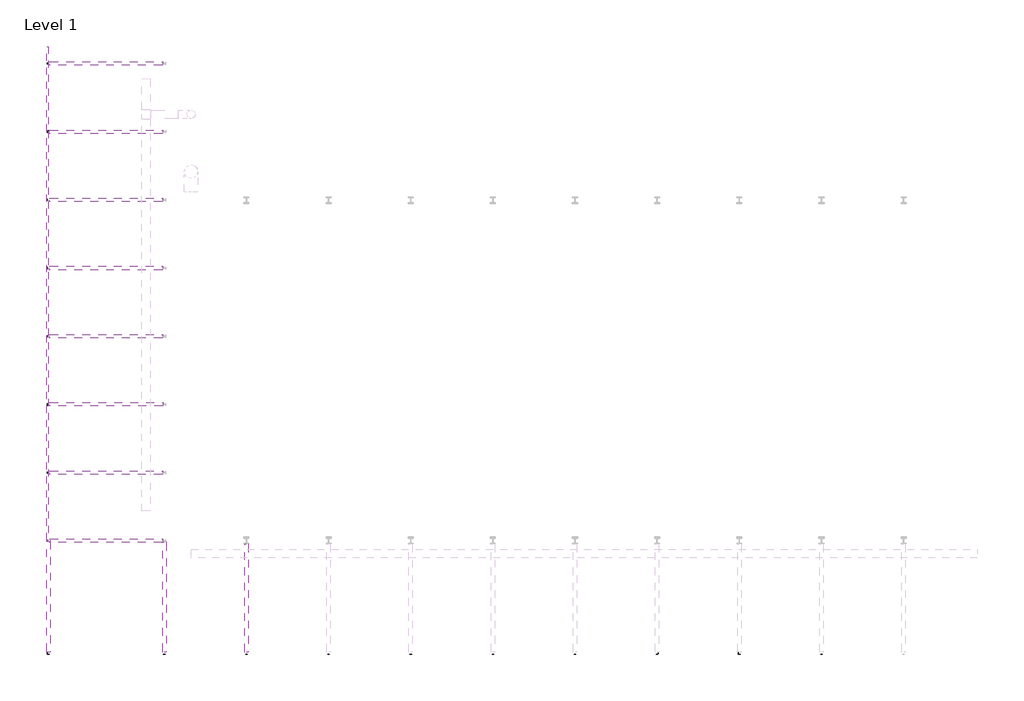
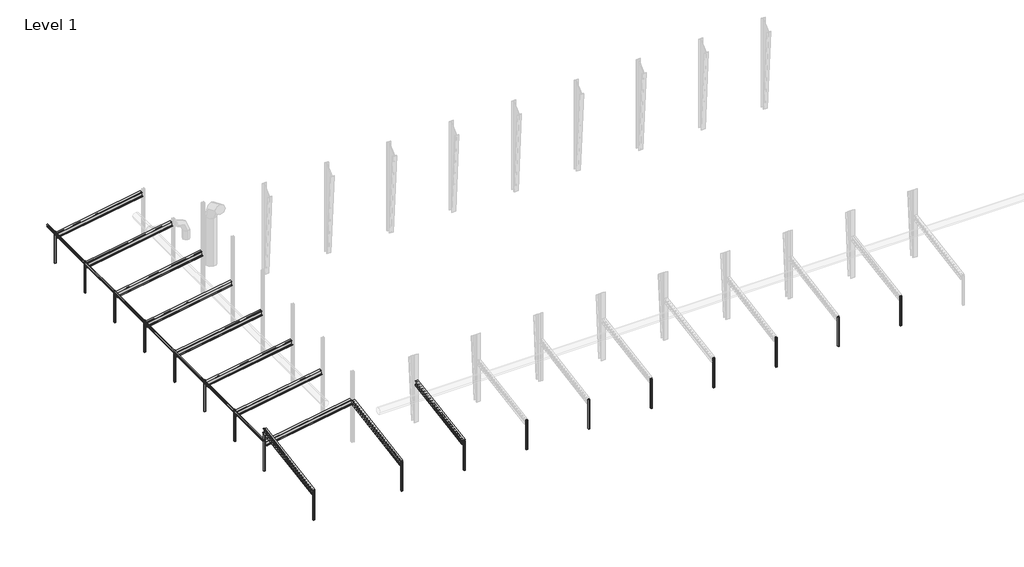
# One storey, part 1 of 3: 18 columns, 12 beams.
"""IFC4 building model written with IfcOpenShell, lengths in millimetres."""

import ifcopenshell
import ifcopenshell.guid

model = None  # the IFC model being written
_history = None  # IfcOwnerHistory: only IFC2X3 demands one
_inside = {}  # id of a spatial element -> (the spatial element, [elements in it])
_under = {}  # id of a project, library or spatial element -> (it, [spatial elements below it])
_declared = {}  # id of a project -> (the project, [libraries it declares])
_typed = {}  # id of a type object -> (the type object, [elements of that type])
_made_of = {}  # id of a material, layer set ... -> (it, [elements and type objects made of it])


def new_model(schema):
    """Start an empty IFC model of exactly this schema.

    Asked for "IFC4X3", IfcOpenShell would pick the latest addendum, in which some entities
    have other attributes; the version numbers below select the first issue.
    IFC2X3 requires an IfcOwnerHistory on every rooted entity: one is made here for all.
    """
    global model, _history
    if schema == "IFC4X3":
        model = ifcopenshell.file(schema_version=(4, 3, 0, 0))
    else:
        model = ifcopenshell.file(schema=schema)
    _inside.clear()
    _under.clear()
    _declared.clear()
    _typed.clear()
    _made_of.clear()
    _history = None
    if model.schema == "IFC2X3":
        org = make("IfcOrganization", Name="unknown")
        user = make(
            "IfcPersonAndOrganization",
            ThePerson=make("IfcPerson", FamilyName="unknown"),
            TheOrganization=org,
        )
        app = make(
            "IfcApplication",
            ApplicationDeveloper=org,
            Version="unknown",
            ApplicationFullName="unknown",
            ApplicationIdentifier="unknown",
        )
        _history = make(
            "IfcOwnerHistory",
            OwningUser=user,
            OwningApplication=app,
            ChangeAction="ADDED",
            CreationDate=0,
        )
    return model


def make(cls, **values):
    """One entity of the class cls with the attributes given. An attribute that is None is left unset."""
    return model.create_entity(
        cls, **{name: value for name, value in values.items() if value is not None}
    )


def rooted(cls, **values):
    """An entity with a GlobalId (a new one), such as an element, a storey or a relation."""
    return make(cls, GlobalId=ifcopenshell.guid.new(), OwnerHistory=_history, **values)


def si_unit(unit_type, name, prefix=None):
    """IfcSIUnit, for example si_unit("LENGTHUNIT", "METRE", prefix="MILLI")."""
    return make("IfcSIUnit", UnitType=unit_type, Prefix=prefix, Name=name)


def assignment(units):
    """IfcUnitAssignment: the units of a project."""
    return None if units is None else make("IfcUnitAssignment", Units=units)


def point(xyz):
    """IfcCartesianPoint."""
    return None if xyz is None else make("IfcCartesianPoint", Coordinates=xyz)


def direction(xyz):
    """IfcDirection."""
    return None if xyz is None else make("IfcDirection", DirectionRatios=xyz)


def frame(location, z_axis=None, x_axis=None):
    """IfcAxis2Placement3D, a coordinate frame: its origin and axes. An axis left out is left unset."""
    return make(
        "IfcAxis2Placement3D",
        Location=point(location),
        Axis=direction(z_axis),
        RefDirection=direction(x_axis),
    )


def frame_2d(location, x_axis=None):
    """IfcAxis2Placement2D, a coordinate frame in the plane: its origin and x axis."""
    return make(
        "IfcAxis2Placement2D", Location=point(location), RefDirection=direction(x_axis)
    )


def origin():
    """The frame at (0, 0, 0) with its axes left unset."""
    return frame((0.0, 0.0, 0.0))


def origin_with_axes():
    """The frame at (0, 0, 0) with the z axis (0, 0, 1) and the x axis (1, 0, 0) written out."""
    return frame((0.0, 0.0, 0.0), z_axis=(0.0, 0.0, 1.0), x_axis=(1.0, 0.0, 0.0))


def place(relative_to, where):
    """IfcLocalPlacement: puts the frame where relative to a parent placement (None: the world)."""
    return make(
        "IfcLocalPlacement", PlacementRelTo=relative_to, RelativePlacement=where
    )


def context(
    kind, dimensions, precision=None, world=None, true_north=None, identifier=None
):
    """IfcGeometricRepresentationContext, for example the 3D "Model" context."""
    return make(
        "IfcGeometricRepresentationContext",
        ContextIdentifier=identifier,
        ContextType=kind,
        CoordinateSpaceDimension=dimensions,
        Precision=precision,
        WorldCoordinateSystem=world,
        TrueNorth=true_north,
    )


def project(units=None, contexts=None):
    """IfcProject with its units and contexts."""
    return rooted(
        "IfcProject",
        Name="project",
        RepresentationContexts=contexts,
        UnitsInContext=assignment(units),
    )


def spatial(cls, under=None, at=None, **own):
    """A site, building, storey or space (cls), placed at a placement, below another one or the project."""
    s = rooted(cls, ObjectPlacement=at, **own)
    if under is not None:
        _under.setdefault(under.id(), (under, []))[1].append(s)
    return s


def polyline(points):
    """IfcPolyline through the points."""
    return make("IfcPolyline", Points=[point(p) for p in points])


def circle_curve(where, radius):
    """IfcCircle in the frame where."""
    return make("IfcCircle", Position=where, Radius=radius)


def trimmed(basis, trim1, trim2, sense, master):
    """IfcTrimmedCurve: the piece of a basis curve between two trims."""
    return make(
        "IfcTrimmedCurve",
        BasisCurve=basis,
        Trim1=trim1,
        Trim2=trim2,
        SenseAgreement=sense,
        MasterRepresentation=master,
    )


def segment(curve, same_sense, transition):
    """IfcCompositeCurveSegment."""
    return make(
        "IfcCompositeCurveSegment",
        Transition=transition,
        SameSense=same_sense,
        ParentCurve=curve,
    )


def composite_curve(segments, self_intersect=None):
    """IfcCompositeCurve: segments joined end to end."""
    return make("IfcCompositeCurve", Segments=segments, SelfIntersect=self_intersect)


def outline(outer, holes=None, kind="AREA"):
    """IfcArbitraryClosedProfileDef: a profile drawn as a closed curve; with holes, ...WithVoids."""
    if holes is None:
        return make("IfcArbitraryClosedProfileDef", ProfileType=kind, OuterCurve=outer)
    return make(
        "IfcArbitraryProfileDefWithVoids",
        ProfileType=kind,
        OuterCurve=outer,
        InnerCurves=holes,
    )


def extrude(swept, where, along, depth):
    """IfcExtrudedAreaSolid: the profile swept, set in the frame where, extruded along a direction by depth."""
    return make(
        "IfcExtrudedAreaSolid",
        SweptArea=swept,
        Position=where,
        ExtrudedDirection=direction(along),
        Depth=depth,
    )


def shape(context_of_items, identifier, shape_type, items):
    """IfcShapeRepresentation: the items that make up one representation, for example the "Body"."""
    return make(
        "IfcShapeRepresentation",
        ContextOfItems=context_of_items,
        RepresentationIdentifier=identifier,
        RepresentationType=shape_type,
        Items=items,
    )


def source(mapping_origin, context_of_items, identifier, shape_type, items):
    """IfcRepresentationMap: a shape defined once, which mapped items show again and again."""
    return make(
        "IfcRepresentationMap",
        MappingOrigin=mapping_origin,
        MappedRepresentation=shape(context_of_items, identifier, shape_type, items),
    )


def transform(
    local_origin,
    x_axis=None,
    y_axis=None,
    z_axis=None,
    scale=None,
    scale2=None,
    scale3=None,
    uniform=True,
):
    """IfcCartesianTransformationOperator3D, or its non-uniform kind. x_axis, y_axis, z_axis: its Axis1, 2, 3."""
    if uniform:
        return make(
            "IfcCartesianTransformationOperator3D",
            Axis1=direction(x_axis),
            Axis2=direction(y_axis),
            LocalOrigin=point(local_origin),
            Scale=scale,
            Axis3=direction(z_axis),
        )
    return make(
        "IfcCartesianTransformationOperator3DnonUniform",
        Axis1=direction(x_axis),
        Axis2=direction(y_axis),
        LocalOrigin=point(local_origin),
        Scale=scale,
        Axis3=direction(z_axis),
        Scale2=scale2,
        Scale3=scale3,
    )


def mapped(mapping_source, mapping_target):
    """IfcMappedItem: shows the shape of a source again, moved by a transform."""
    return make(
        "IfcMappedItem", MappingSource=mapping_source, MappingTarget=mapping_target
    )


def made_of(thing, what):
    """Note that an element or type object is made of a material, layer set ...; save() writes the relation."""
    if what is not None:
        _made_of.setdefault(what.id(), (what, []))[1].append(thing)
    return thing


def element(
    cls,
    number,
    at=None,
    inside=None,
    cuts=None,
    type_object=None,
    material=None,
    context=None,
    identifier="Body",
    shape_type=None,
    held_by="IfcProductDefinitionShape",
    body=None,
    shapes=None,
    **own,
):
    """One element of the class cls, such as IfcWall. Its Tag is "e" and its number.

    at: its placement. inside: the storey or other place that contains it. cuts: it is an
    opening in that element (IfcRelVoidsElement). A single representation is given by context,
    identifier, shape_type and body (its items); several are given by shapes. held_by: the class
    of the entity that holds the representations. save() writes the other relations.
    """
    e = rooted(cls, Tag="e%d" % number, ObjectPlacement=at, **own)
    if body is not None:
        shapes = [shape(context, identifier, shape_type, body)]
    if shapes is not None:
        e.Representation = make(held_by, Representations=shapes)
    if inside is not None:
        _inside.setdefault(inside.id(), (inside, []))[1].append(e)
    if cuts is not None:
        rooted(
            "IfcRelVoidsElement", RelatingBuildingElement=cuts, RelatedOpeningElement=e
        )
    if type_object is not None:
        _typed.setdefault(type_object.id(), (type_object, []))[1].append(e)
    return made_of(e, material)


def aggregate(whole, parts):
    """IfcRelAggregates: a whole, such as a stair, and the parts it consists of."""
    return rooted("IfcRelAggregates", RelatingObject=whole, RelatedObjects=parts)


def save(model, path):
    """Write the relations noted so far, then the file.

    IfcRelAggregates (storeys below a building ...), IfcRelContainedInSpatialStructure (elements
    in a storey), IfcRelDefinesByType, IfcRelAssociatesMaterial and IfcRelDeclares: one each for
    every whole, place, type object, material and project.
    """
    for whole, parts in _under.values():
        aggregate(whole, parts)
    for where, things in _inside.values():
        rooted(
            "IfcRelContainedInSpatialStructure",
            RelatedElements=things,
            RelatingStructure=where,
        )
    for kind, things in _typed.values():
        rooted("IfcRelDefinesByType", RelatedObjects=things, RelatingType=kind)
    for what, things in _made_of.values():
        rooted("IfcRelAssociatesMaterial", RelatedObjects=things, RelatingMaterial=what)
    for by, libraries in _declared.values():
        rooted("IfcRelDeclares", RelatingContext=by, RelatedDefinitions=libraries)
    model.write(path)


def beam_fa991611(model_context):
    return source(origin(), model_context, "Body", "SweptSolid", [
        extrude(outline(composite_curve([segment(polyline([(63.5, 127.0), (75.745104, 112.4068534), (73.6169367, 110.621109), (62.204539, 124.221875), (3.3005807, 124.221875)]), True, "CONTINUOUS"), segment(trimmed(circle_curve(frame_2d((3.3741066, 122.2381931)), 1.9850441), [point((3.3005807, 124.221875))], [point((1.3890625, 122.2381931))], True, "CARTESIAN"), True, "CONTINUOUS"), segment(polyline([(1.3890625, 122.2381931), (1.3890625, -122.2375)]), True, "CONTINUOUS"), segment(trimmed(circle_curve(frame_2d((-3.3734375, -122.2375)), 4.7625), [point((1.3890625, -122.2375))], [point((-3.3734375, -127.0))], False, "CARTESIAN"), True, "CONTINUOUS"), segment(polyline([(-3.3734375, -127.0), (-63.5, -127.0), (-75.745104, -112.4068534), (-73.6169367, -110.621109), (-62.204539, -124.221875), (-3.2694106, -124.221875)]), True, "CONTINUOUS"), segment(trimmed(circle_curve(frame_2d((-3.3748024, -122.2389339)), 1.9857399), [point((-3.2694106, -124.221875))], [point((-1.3890625, -122.2389339))], True, "CARTESIAN"), True, "CONTINUOUS"), segment(polyline([(-1.3890625, -122.2389339), (-1.3890625, 122.2375)]), True, "CONTINUOUS"), segment(trimmed(circle_curve(frame_2d((3.3734375, 122.2375)), 4.7625), [point((-1.3890625, 122.2375))], [point((3.3734375, 127.0))], False, "CARTESIAN"), True, "CONTINUOUS"), segment(polyline([(3.3734375, 127.0), (63.5, 127.0)]), True, "CONTINUOUS")], self_intersect=False)), frame((-22098.0, 0.0, 0.0), z_axis=(1.0, 0.0, 0.0), x_axis=(0.0, 1.0, 0.0)), (0.0, 0.0, 1.0), 44107.1),
    ])


def w_wide_flange_w21x166_c1e76bd8(model_context):
    return source(origin(), model_context, "Body", "SweptSolid", [
        extrude(outline(composite_curve([segment(polyline([(157.48, -251.206), (157.48, -285.75), (-157.48, -285.75), (-157.48, -251.206), (-32.131, -251.206)]), True, "CONTINUOUS"), segment(trimmed(circle_curve(frame_2d((-32.131, -228.6)), 22.606), [point((-32.131, -251.206))], [point((-9.525, -228.6))], True, "CARTESIAN"), True, "CONTINUOUS"), segment(polyline([(-9.525, -228.6), (-9.525, 228.6)]), True, "CONTINUOUS"), segment(trimmed(circle_curve(frame_2d((-32.131, 228.6)), 22.606), [point((-9.525, 228.6))], [point((-32.131, 251.206))], True, "CARTESIAN"), True, "CONTINUOUS"), segment(polyline([(-32.131, 251.206), (-157.48, 251.206), (-157.48, 285.75), (157.48, 285.75), (157.48, 251.206), (32.131, 251.206)]), True, "CONTINUOUS"), segment(trimmed(circle_curve(frame_2d((32.131, 228.6)), 22.606), [point((32.131, 251.206))], [point((9.525, 228.6))], True, "CARTESIAN"), True, "CONTINUOUS"), segment(polyline([(9.525, 228.6), (9.525, -228.6)]), True, "CONTINUOUS"), segment(trimmed(circle_curve(frame_2d((32.131, -228.6)), 22.606), [point((9.525, -228.6))], [point((32.131, -251.206))], True, "CARTESIAN"), True, "CONTINUOUS"), segment(polyline([(32.131, -251.206), (157.48, -251.206)]), True, "CONTINUOUS")], self_intersect=False)), frame((-4963.0833359, 0.0, 0.0), z_axis=(1.0, 0.0, 0.0), x_axis=(0.0, 1.0, 0.0)), (0.0, 0.0, 1.0), 9743.826275),
    ])


def w_wide_flange_w21x166_98a64792(model_context):
    return source(origin(), model_context, "Body", "SweptSolid", [
        extrude(outline(composite_curve([segment(polyline([(157.48, -251.206), (157.48, -285.75), (-157.48, -285.75), (-157.48, -251.206), (-32.131, -251.206)]), True, "CONTINUOUS"), segment(trimmed(circle_curve(frame_2d((-32.131, -228.6)), 22.606), [point((-32.131, -251.206))], [point((-9.525, -228.6))], True, "CARTESIAN"), True, "CONTINUOUS"), segment(polyline([(-9.525, -228.6), (-9.525, 228.6)]), True, "CONTINUOUS"), segment(trimmed(circle_curve(frame_2d((-32.131, 228.6)), 22.606), [point((-9.525, 228.6))], [point((-32.131, 251.206))], True, "CARTESIAN"), True, "CONTINUOUS"), segment(polyline([(-32.131, 251.206), (-157.48, 251.206), (-157.48, 285.75), (157.48, 285.75), (157.48, 251.206), (32.131, 251.206)]), True, "CONTINUOUS"), segment(trimmed(circle_curve(frame_2d((32.131, 228.6)), 22.606), [point((32.131, 251.206))], [point((9.525, 228.6))], True, "CARTESIAN"), True, "CONTINUOUS"), segment(polyline([(9.525, 228.6), (9.525, -228.6)]), True, "CONTINUOUS"), segment(trimmed(circle_curve(frame_2d((32.131, -228.6)), 22.606), [point((9.525, -228.6))], [point((32.131, -251.206))], True, "CARTESIAN"), True, "CONTINUOUS"), segment(polyline([(32.131, -251.206), (157.48, -251.206)]), True, "CONTINUOUS")], self_intersect=False)), frame((-4963.0833357, 0.0, 0.0), z_axis=(1.0, 0.0, 0.0), x_axis=(0.0, 1.0, 0.0)), (0.0, 0.0, 1.0), 10061.6548886),
    ])


def w_wide_flange_w21x166_1b8c9151(model_context):
    return source(origin(), model_context, "Body", "SweptSolid", [
        extrude(outline(composite_curve([segment(polyline([(157.48, -251.206), (157.48, -285.75), (-157.48, -285.75), (-157.48, -251.206), (-32.131, -251.206)]), True, "CONTINUOUS"), segment(trimmed(circle_curve(frame_2d((-32.131, -228.6)), 22.606), [point((-32.131, -251.206))], [point((-9.525, -228.6))], True, "CARTESIAN"), True, "CONTINUOUS"), segment(polyline([(-9.525, -228.6), (-9.525, 228.6)]), True, "CONTINUOUS"), segment(trimmed(circle_curve(frame_2d((-32.131, 228.6)), 22.606), [point((-9.525, 228.6))], [point((-32.131, 251.206))], True, "CARTESIAN"), True, "CONTINUOUS"), segment(polyline([(-32.131, 251.206), (-157.48, 251.206), (-157.48, 285.75), (157.48, 285.75), (157.48, 251.206), (32.131, 251.206)]), True, "CONTINUOUS"), segment(trimmed(circle_curve(frame_2d((32.131, 228.6)), 22.606), [point((32.131, 251.206))], [point((9.525, 228.6))], True, "CARTESIAN"), True, "CONTINUOUS"), segment(polyline([(9.525, 228.6), (9.525, -228.6)]), True, "CONTINUOUS"), segment(trimmed(circle_curve(frame_2d((32.131, -228.6)), 22.606), [point((9.525, -228.6))], [point((32.131, -251.206))], True, "CARTESIAN"), True, "CONTINUOUS"), segment(polyline([(32.131, -251.206), (157.48, -251.206)]), True, "CONTINUOUS")], self_intersect=False)), frame((-4963.0833359, 0.0, 0.0), z_axis=(1.0, 0.0, 0.0), x_axis=(0.0, 1.0, 0.0)), (0.0, 0.0, 1.0), 9898.83138),
    ])


def w_wide_flange_w21x166_41bf6792(model_context):
    return source(origin(), model_context, "Body", "SweptSolid", [
        extrude(outline(composite_curve([segment(polyline([(157.48, -251.206), (157.48, -285.75), (-157.48, -285.75), (-157.48, -251.206), (-32.131, -251.206)]), True, "CONTINUOUS"), segment(trimmed(circle_curve(frame_2d((-32.131, -228.6)), 22.606), [point((-32.131, -251.206))], [point((-9.525, -228.6))], True, "CARTESIAN"), True, "CONTINUOUS"), segment(polyline([(-9.525, -228.6), (-9.525, 228.6)]), True, "CONTINUOUS"), segment(trimmed(circle_curve(frame_2d((-32.131, 228.6)), 22.606), [point((-9.525, 228.6))], [point((-32.131, 251.206))], True, "CARTESIAN"), True, "CONTINUOUS"), segment(polyline([(-32.131, 251.206), (-157.48, 251.206), (-157.48, 285.75), (157.48, 285.75), (157.48, 251.206), (32.131, 251.206)]), True, "CONTINUOUS"), segment(trimmed(circle_curve(frame_2d((32.131, 228.6)), 22.606), [point((32.131, 251.206))], [point((9.525, 228.6))], True, "CARTESIAN"), True, "CONTINUOUS"), segment(polyline([(9.525, 228.6), (9.525, -228.6)]), True, "CONTINUOUS"), segment(trimmed(circle_curve(frame_2d((32.131, -228.6)), 22.606), [point((9.525, -228.6))], [point((32.131, -251.206))], True, "CARTESIAN"), True, "CONTINUOUS"), segment(polyline([(32.131, -251.206), (157.48, -251.206)]), True, "CONTINUOUS")], self_intersect=False)), frame((-5180.0235462, 0.0, 0.0), z_axis=(1.0, 0.0, 0.0), x_axis=(0.0, 1.0, 0.0)), (0.0, 0.0, 1.0), 10224.7221576),
    ])


def w_wide_flange_w21x166_82cd9a53(model_context):
    return source(origin(), model_context, "Body", "SweptSolid", [
        extrude(outline(composite_curve([segment(polyline([(157.48, -251.206), (157.48, -285.75), (-157.48, -285.75), (-157.48, -251.206), (-32.131, -251.206)]), True, "CONTINUOUS"), segment(trimmed(circle_curve(frame_2d((-32.131, -228.6)), 22.606), [point((-32.131, -251.206))], [point((-9.525, -228.6))], True, "CARTESIAN"), True, "CONTINUOUS"), segment(polyline([(-9.525, -228.6), (-9.525, 228.6)]), True, "CONTINUOUS"), segment(trimmed(circle_curve(frame_2d((-32.131, 228.6)), 22.606), [point((-9.525, 228.6))], [point((-32.131, 251.206))], True, "CARTESIAN"), True, "CONTINUOUS"), segment(polyline([(-32.131, 251.206), (-157.48, 251.206), (-157.48, 285.75), (157.48, 285.75), (157.48, 251.206), (32.131, 251.206)]), True, "CONTINUOUS"), segment(trimmed(circle_curve(frame_2d((32.131, 228.6)), 22.606), [point((32.131, 251.206))], [point((9.525, 228.6))], True, "CARTESIAN"), True, "CONTINUOUS"), segment(polyline([(9.525, 228.6), (9.525, -228.6)]), True, "CONTINUOUS"), segment(trimmed(circle_curve(frame_2d((32.131, -228.6)), 22.606), [point((9.525, -228.6))], [point((32.131, -251.206))], True, "CARTESIAN"), True, "CONTINUOUS"), segment(polyline([(32.131, -251.206), (157.48, -251.206)]), True, "CONTINUOUS")], self_intersect=False)), frame((-5180.0235462, 0.0, 0.0), z_axis=(1.0, 0.0, 0.0), x_axis=(0.0, 1.0, 0.0)), (0.0, 0.0, 1.0), 10182.9648149),
    ])


def hss_hollow_structural_section_column_hss6x6x1_4_de73236b(model_context):
    return source(origin(), model_context, "Body", "SweptSolid", [
        extrude(outline(composite_curve([segment(trimmed(circle_curve(frame_2d((64.3636, 64.3636)), 11.8364), [point((64.3636, 76.2))], [point((76.2, 64.3636))], False, "CARTESIAN"), True, "CONTINUOUS"), segment(polyline([(76.2, 64.3636), (76.2, -64.3636)]), True, "CONTINUOUS"), segment(trimmed(circle_curve(frame_2d((64.3636, -64.3636)), 11.8364), [point((76.2, -64.3636))], [point((64.3636, -76.2))], False, "CARTESIAN"), True, "CONTINUOUS"), segment(polyline([(64.3636, -76.2), (-64.3636, -76.2)]), True, "CONTINUOUS"), segment(trimmed(circle_curve(frame_2d((-64.3636, -64.3636)), 11.8364), [point((-64.3636, -76.2))], [point((-76.2, -64.3636))], False, "CARTESIAN"), True, "CONTINUOUS"), segment(polyline([(-76.2, -64.3636), (-76.2, 64.3636)]), True, "CONTINUOUS"), segment(trimmed(circle_curve(frame_2d((-64.3636, 64.3636)), 11.8364), [point((-76.2, 64.3636))], [point((-64.3636, 76.2))], False, "CARTESIAN"), True, "CONTINUOUS"), segment(polyline([(-64.3636, 76.2), (64.3636, 76.2)]), True, "CONTINUOUS")], self_intersect=False), holes=[composite_curve([segment(polyline([(64.3636, 70.2818), (-64.3636, 70.2818)]), True, "CONTINUOUS"), segment(trimmed(circle_curve(frame_2d((-64.3636, 64.3636)), 5.9182), [point((-64.3636, 70.2818))], [point((-70.2818, 64.3636))], True, "CARTESIAN"), True, "CONTINUOUS"), segment(polyline([(-70.2818, 64.3636), (-70.2818, -64.3636)]), True, "CONTINUOUS"), segment(trimmed(circle_curve(frame_2d((-64.3636, -64.3636)), 5.9182), [point((-70.2818, -64.3636))], [point((-64.3636, -70.2818))], True, "CARTESIAN"), True, "CONTINUOUS"), segment(polyline([(-64.3636, -70.2818), (64.3636, -70.2818)]), True, "CONTINUOUS"), segment(trimmed(circle_curve(frame_2d((64.3636, -64.3636)), 5.9182), [point((64.3636, -70.2818))], [point((70.2818, -64.3636))], True, "CARTESIAN"), True, "CONTINUOUS"), segment(polyline([(70.2818, -64.3636), (70.2818, 64.3636)]), True, "CONTINUOUS"), segment(trimmed(circle_curve(frame_2d((64.3636, 64.3636)), 5.9182), [point((70.2818, 64.3636))], [point((64.3636, 70.2818))], True, "CARTESIAN"), True, "CONTINUOUS")], self_intersect=False)]), origin_with_axes(), (0.0, 0.0, 1.0), 3657.6),
    ])


model = new_model("IFC4")

# Units and contexts
model_context = context("Model", 3, world=origin())
ifc_project = project(units=[si_unit("LENGTHUNIT", "METRE", prefix="MILLI")], contexts=[model_context])

# Site, building, storey
site = spatial("IfcSite", under=ifc_project)
building = spatial("IfcBuilding", under=site)
storey = spatial("IfcBuildingStorey", under=building, Name="Level 1", Elevation=0.0)

# Beams
placement = place(None, origin())
beam_shape = beam_fa991611(model_context)
element("IfcBeam", 1, ObjectType="Girt_Z : 10\"D", at=placement, inside=storey, context=model_context, shape_type="MappedRepresentation", body=[
    mapped(beam_shape, transform((568593.9120802, -545593.3413841, 3774.4851996), x_axis=(0.0, -1.0, 0.0), y_axis=(0.986393923832142, 0.0, 0.16439898730536787), z_axis=(-0.16439898730536787, 0.0, 0.986393923832142))),
])
w_wide_flange_w21x166_shape = w_wide_flange_w21x166_c1e76bd8(model_context)
element("IfcBeam", 2, ObjectType="W-Wide Flange : W21X166", at=placement, inside=storey, context=model_context, shape_type="MappedRepresentation", body=[
    mapped(w_wide_flange_w21x166_shape, transform((586368.911724, -572720.5413841, 4206.1084345), x_axis=(0.0, 0.9863939238321447, 0.16439898730535185), y_axis=(-1.0000000000000002, 0.0, 0.0), z_axis=(0.0, -0.16439898730535224, 0.9863939238321446))),
])
w_wide_flange_w21x166_2_shape = w_wide_flange_w21x166_98a64792(model_context)
element("IfcBeam", 3, ObjectType="W-Wide Flange : W21X166", at=placement, inside=storey, context=model_context, shape_type="MappedRepresentation", body=[
    mapped(w_wide_flange_w21x166_2_shape, transform((568665.111724, -572720.5413841, 4206.1084345), x_axis=(0.0, 0.9863939238321447, 0.16439898730535185), y_axis=(-1.0000000000000002, 0.0, 0.0), z_axis=(0.0, -0.16439898730535224, 0.9863939238321446))),
])
w_wide_flange_w21x166_3_shape = w_wide_flange_w21x166_1b8c9151(model_context)
element("IfcBeam", 4, ObjectType="W-Wide Flange : W21X166", at=placement, inside=storey, context=model_context, shape_type="MappedRepresentation", body=[
    mapped(w_wide_flange_w21x166_3_shape, transform((579028.311724, -572720.5413841, 4206.1084345), x_axis=(0.0, 0.9863939238321447, 0.16439898730535185), y_axis=(-1.0000000000000002, 0.0, 0.0), z_axis=(0.0, -0.16439898730535218, 0.9863939238321446))),
])
w_wide_flange_w21x166_4_shape = w_wide_flange_w21x166_41bf6792(model_context)
element("IfcBeam", 5, ObjectType="W-Wide Flange : W21X166", at=placement, inside=storey, context=model_context, shape_type="MappedRepresentation", body=[
    mapped(w_wide_flange_w21x166_4_shape, transform((573910.3596887, -555499.3413841, 4242.1164286), x_axis=(0.9863939238321418, 0.0, 0.1643989873053695), y_axis=(0.0, 1.0, 0.0), z_axis=(-0.16439898730536961, 0.0, 0.9863939238321418))),
])
w_wide_flange_w21x166_5_shape = w_wide_flange_w21x166_82cd9a53(model_context)
element("IfcBeam", 6, ObjectType="W-Wide Flange : W21X166", at=placement, inside=storey, context=model_context, shape_type="MappedRepresentation", body=[
    mapped(w_wide_flange_w21x166_5_shape, transform((573910.3596887, -549403.3413841, 4242.1164286), x_axis=(0.9863939238321418, 0.0, 0.1643989873053695), y_axis=(0.0, 1.0, 0.0), z_axis=(-0.16439898730536961, 0.0, 0.9863939238321418))),
])
element("IfcBeam", 7, ObjectType="W-Wide Flange : W21X166", at=placement, inside=storey, context=model_context, shape_type="MappedRepresentation", body=[
    mapped(w_wide_flange_w21x166_5_shape, transform((573910.3596887, -543307.3413841, 4242.1164286), x_axis=(0.9863939238321418, 0.0, 0.1643989873053695), y_axis=(0.0, 1.0, 0.0), z_axis=(-0.16439898730536961, 0.0, 0.9863939238321418))),
])
element("IfcBeam", 8, ObjectType="W-Wide Flange : W21X166", at=placement, inside=storey, context=model_context, shape_type="MappedRepresentation", body=[
    mapped(w_wide_flange_w21x166_5_shape, transform((573910.3596887, -537211.3413841, 4242.1164286), x_axis=(0.9863939238321418, 0.0, 0.1643989873053695), y_axis=(0.0, 1.0, 0.0), z_axis=(-0.16439898730536961, 0.0, 0.9863939238321418))),
])
element("IfcBeam", 9, ObjectType="W-Wide Flange : W21X166", at=placement, inside=storey, context=model_context, shape_type="MappedRepresentation", body=[
    mapped(w_wide_flange_w21x166_5_shape, transform((573910.3596887, -531115.3413841, 4242.1164286), x_axis=(0.9863939238321418, 0.0, 0.1643989873053695), y_axis=(0.0, 1.0, 0.0), z_axis=(-0.16439898730536961, 0.0, 0.9863939238321418))),
])
element("IfcBeam", 10, ObjectType="W-Wide Flange : W21X166", at=placement, inside=storey, context=model_context, shape_type="MappedRepresentation", body=[
    mapped(w_wide_flange_w21x166_5_shape, transform((573910.3596887, -525019.3413841, 4242.1164286), x_axis=(0.9863939238321418, 0.0, 0.1643989873053695), y_axis=(0.0, 1.0, 0.0), z_axis=(-0.16439898730536961, 0.0, 0.9863939238321418))),
])
element("IfcBeam", 11, ObjectType="W-Wide Flange : W21X166", at=placement, inside=storey, context=model_context, shape_type="MappedRepresentation", body=[
    mapped(w_wide_flange_w21x166_5_shape, transform((573910.3596887, -561595.3413841, 4242.1164286), x_axis=(0.9863939238321418, 0.0, 0.1643989873053695), y_axis=(0.0, 1.0, 0.0), z_axis=(-0.16439898730536961, 0.0, 0.9863939238321418))),
])
element("IfcBeam", 12, ObjectType="W-Wide Flange : W21X166", at=placement, inside=storey, context=model_context, shape_type="MappedRepresentation", body=[
    mapped(w_wide_flange_w21x166_5_shape, transform((573910.3596887, -567691.3413841, 4242.1164286), x_axis=(0.9863939238321418, 0.0, 0.1643989873053695), y_axis=(0.0, 1.0, 0.0), z_axis=(-0.16439898730536961, 0.0, 0.9863939238321418))),
])

# Columns
element("IfcColumn", 13, ObjectType="HSS-Hollow Structural Section-Column : HSS6X6X1/4", at=placement, inside=storey, context=model_context, shape_type="SweptSolid", body=[
    extrude(outline(composite_curve([segment(trimmed(circle_curve(frame_2d((568729.4753239, -567755.7049841)), 11.8364), [point((568741.3117239, -567755.7049841))], [point((568729.4753239, -567767.5413841))], False, "CARTESIAN"), True, "CONTINUOUS"), segment(polyline([(568729.4753239, -567767.5413841), (568600.7481239, -567767.5413841)]), True, "CONTINUOUS"), segment(trimmed(circle_curve(frame_2d((568600.7481239, -567755.7049841)), 11.8364), [point((568600.7481239, -567767.5413841))], [point((568588.9117239, -567755.7049841))], False, "CARTESIAN"), True, "CONTINUOUS"), segment(polyline([(568588.9117239, -567755.7049841), (568588.9117239, -567626.9777841)]), True, "CONTINUOUS"), segment(trimmed(circle_curve(frame_2d((568600.7481239, -567626.9777841)), 11.8364), [point((568588.9117239, -567626.9777841))], [point((568600.7481239, -567615.1413841))], False, "CARTESIAN"), True, "CONTINUOUS"), segment(polyline([(568600.7481239, -567615.1413841), (568729.4753239, -567615.1413841)]), True, "CONTINUOUS"), segment(trimmed(circle_curve(frame_2d((568729.4753239, -567626.9777841)), 11.8364), [point((568729.4753239, -567615.1413841))], [point((568741.3117239, -567626.9777841))], False, "CARTESIAN"), True, "CONTINUOUS"), segment(polyline([(568741.3117239, -567626.9777841), (568741.3117239, -567755.7049841)]), True, "CONTINUOUS")], self_intersect=False), holes=[composite_curve([segment(polyline([(568735.3935239, -567755.7049841), (568735.3935239, -567626.9777841)]), True, "CONTINUOUS"), segment(trimmed(circle_curve(frame_2d((568729.4753239, -567626.9777841)), 5.9182), [point((568735.3935239, -567626.9777841))], [point((568729.4753239, -567621.0595841))], True, "CARTESIAN"), True, "CONTINUOUS"), segment(polyline([(568729.4753239, -567621.0595841), (568600.7481239, -567621.0595841)]), True, "CONTINUOUS"), segment(trimmed(circle_curve(frame_2d((568600.7481239, -567626.9777841)), 5.9182), [point((568600.7481239, -567621.0595841))], [point((568594.8299239, -567626.9777841))], True, "CARTESIAN"), True, "CONTINUOUS"), segment(polyline([(568594.8299239, -567626.9777841), (568594.8299239, -567755.7049841)]), True, "CONTINUOUS"), segment(trimmed(circle_curve(frame_2d((568600.7481239, -567755.7049841)), 5.9182), [point((568594.8299239, -567755.7049841))], [point((568600.7481239, -567761.6231841))], True, "CARTESIAN"), True, "CONTINUOUS"), segment(polyline([(568600.7481239, -567761.6231841), (568729.4753239, -567761.6231841)]), True, "CONTINUOUS"), segment(trimmed(circle_curve(frame_2d((568729.4753239, -567755.7049841)), 5.9182), [point((568729.4753239, -567761.6231841))], [point((568735.3935239, -567755.7049841))], True, "CARTESIAN"), True, "CONTINUOUS")], self_intersect=False)]), origin_with_axes(), (0.0, 0.0, 1.0), 4741.916869),
])
element("IfcColumn", 14, ObjectType="HSS-Hollow Structural Section-Column : HSS6X6X1/4", at=placement, inside=storey, context=model_context, shape_type="SweptSolid", body=[
    extrude(outline(composite_curve([segment(trimmed(circle_curve(frame_2d((568600.7481239, -537275.7049841)), 11.8364), [point((568600.7481239, -537287.5413841))], [point((568588.9117239, -537275.7049841))], False, "CARTESIAN"), True, "CONTINUOUS"), segment(polyline([(568588.9117239, -537275.7049841), (568588.9117239, -537146.9777841)]), True, "CONTINUOUS"), segment(trimmed(circle_curve(frame_2d((568600.7481239, -537146.9777841)), 11.8364), [point((568588.9117239, -537146.9777841))], [point((568600.7481239, -537135.1413841))], False, "CARTESIAN"), True, "CONTINUOUS"), segment(polyline([(568600.7481239, -537135.1413841), (568729.4753239, -537135.1413841)]), True, "CONTINUOUS"), segment(trimmed(circle_curve(frame_2d((568729.4753239, -537146.9777841)), 11.8364), [point((568729.4753239, -537135.1413841))], [point((568741.3117239, -537146.9777841))], False, "CARTESIAN"), True, "CONTINUOUS"), segment(polyline([(568741.3117239, -537146.9777841), (568741.3117239, -537275.7049841)]), True, "CONTINUOUS"), segment(trimmed(circle_curve(frame_2d((568729.4753239, -537275.7049841)), 11.8364), [point((568741.3117239, -537275.7049841))], [point((568729.4753239, -537287.5413841))], False, "CARTESIAN"), True, "CONTINUOUS"), segment(polyline([(568729.4753239, -537287.5413841), (568600.7481239, -537287.5413841)]), True, "CONTINUOUS")], self_intersect=False), holes=[composite_curve([segment(polyline([(568600.7481239, -537281.6231841), (568729.4753239, -537281.6231841)]), True, "CONTINUOUS"), segment(trimmed(circle_curve(frame_2d((568729.4753239, -537275.7049841)), 5.9182), [point((568729.4753239, -537281.6231841))], [point((568735.3935239, -537275.7049841))], True, "CARTESIAN"), True, "CONTINUOUS"), segment(polyline([(568735.3935239, -537275.7049841), (568735.3935239, -537146.9777841)]), True, "CONTINUOUS"), segment(trimmed(circle_curve(frame_2d((568729.4753239, -537146.9777841)), 5.9182), [point((568735.3935239, -537146.9777841))], [point((568729.4753239, -537141.0595841))], True, "CARTESIAN"), True, "CONTINUOUS"), segment(polyline([(568729.4753239, -537141.0595841), (568600.7481239, -537141.0595841)]), True, "CONTINUOUS"), segment(trimmed(circle_curve(frame_2d((568600.7481239, -537146.9777841)), 5.9182), [point((568600.7481239, -537141.0595841))], [point((568594.8299239, -537146.9777841))], True, "CARTESIAN"), True, "CONTINUOUS"), segment(polyline([(568594.8299239, -537146.9777841), (568594.8299239, -537275.7049841)]), True, "CONTINUOUS"), segment(trimmed(circle_curve(frame_2d((568600.7481239, -537275.7049841)), 5.9182), [point((568594.8299239, -537275.7049841))], [point((568600.7481239, -537281.6231841))], True, "CARTESIAN"), True, "CONTINUOUS")], self_intersect=False)]), origin_with_axes(), (0.0, 0.0, 1.0), 3902.4036138),
])
element("IfcColumn", 15, ObjectType="HSS-Hollow Structural Section-Column : HSS6X6X1/4", at=placement, inside=storey, context=model_context, shape_type="SweptSolid", body=[
    extrude(outline(composite_curve([segment(trimmed(circle_curve(frame_2d((568600.7481239, -525083.7049841)), 11.8364), [point((568600.7481239, -525095.5413841))], [point((568588.9117239, -525083.7049841))], False, "CARTESIAN"), True, "CONTINUOUS"), segment(polyline([(568588.9117239, -525083.7049841), (568588.9117239, -524954.9777841)]), True, "CONTINUOUS"), segment(trimmed(circle_curve(frame_2d((568600.7481239, -524954.9777841)), 11.8364), [point((568588.9117239, -524954.9777841))], [point((568600.7481239, -524943.1413841))], False, "CARTESIAN"), True, "CONTINUOUS"), segment(polyline([(568600.7481239, -524943.1413841), (568729.4753239, -524943.1413841)]), True, "CONTINUOUS"), segment(trimmed(circle_curve(frame_2d((568729.4753239, -524954.9777841)), 11.8364), [point((568729.4753239, -524943.1413841))], [point((568741.3117239, -524954.9777841))], False, "CARTESIAN"), True, "CONTINUOUS"), segment(polyline([(568741.3117239, -524954.9777841), (568741.3117239, -525083.7049841)]), True, "CONTINUOUS"), segment(trimmed(circle_curve(frame_2d((568729.4753239, -525083.7049841)), 11.8364), [point((568741.3117239, -525083.7049841))], [point((568729.4753239, -525095.5413841))], False, "CARTESIAN"), True, "CONTINUOUS"), segment(polyline([(568729.4753239, -525095.5413841), (568600.7481239, -525095.5413841)]), True, "CONTINUOUS")], self_intersect=False), holes=[composite_curve([segment(polyline([(568600.7481239, -525089.6231841), (568729.4753239, -525089.6231841)]), True, "CONTINUOUS"), segment(trimmed(circle_curve(frame_2d((568729.4753239, -525083.7049841)), 5.9182), [point((568729.4753239, -525089.6231841))], [point((568735.3935239, -525083.7049841))], True, "CARTESIAN"), True, "CONTINUOUS"), segment(polyline([(568735.3935239, -525083.7049841), (568735.3935239, -524954.9777841)]), True, "CONTINUOUS"), segment(trimmed(circle_curve(frame_2d((568729.4753239, -524954.9777841)), 5.9182), [point((568735.3935239, -524954.9777841))], [point((568729.4753239, -524949.0595841))], True, "CARTESIAN"), True, "CONTINUOUS"), segment(polyline([(568729.4753239, -524949.0595841), (568600.7481239, -524949.0595841)]), True, "CONTINUOUS"), segment(trimmed(circle_curve(frame_2d((568600.7481239, -524954.9777841)), 5.9182), [point((568600.7481239, -524949.0595841))], [point((568594.8299239, -524954.9777841))], True, "CARTESIAN"), True, "CONTINUOUS"), segment(polyline([(568594.8299239, -524954.9777841), (568594.8299239, -525083.7049841)]), True, "CONTINUOUS"), segment(trimmed(circle_curve(frame_2d((568600.7481239, -525083.7049841)), 5.9182), [point((568594.8299239, -525083.7049841))], [point((568600.7481239, -525089.6231841))], True, "CARTESIAN"), True, "CONTINUOUS")], self_intersect=False)]), origin_with_axes(), (0.0, 0.0, 1.0), 3902.4036138),
])
element("IfcColumn", 16, ObjectType="HSS-Hollow Structural Section-Column : HSS6X6X1/4", at=placement, inside=storey, context=model_context, shape_type="SweptSolid", body=[
    extrude(outline(composite_curve([segment(trimmed(circle_curve(frame_2d((568600.7481239, -543371.7049841)), 11.8364), [point((568600.7481239, -543383.5413841))], [point((568588.9117239, -543371.7049841))], False, "CARTESIAN"), True, "CONTINUOUS"), segment(polyline([(568588.9117239, -543371.7049841), (568588.9117239, -543242.9777841)]), True, "CONTINUOUS"), segment(trimmed(circle_curve(frame_2d((568600.7481239, -543242.9777841)), 11.8364), [point((568588.9117239, -543242.9777841))], [point((568600.7481239, -543231.1413841))], False, "CARTESIAN"), True, "CONTINUOUS"), segment(polyline([(568600.7481239, -543231.1413841), (568729.4753239, -543231.1413841)]), True, "CONTINUOUS"), segment(trimmed(circle_curve(frame_2d((568729.4753239, -543242.9777841)), 11.8364), [point((568729.4753239, -543231.1413841))], [point((568741.3117239, -543242.9777841))], False, "CARTESIAN"), True, "CONTINUOUS"), segment(polyline([(568741.3117239, -543242.9777841), (568741.3117239, -543371.7049841)]), True, "CONTINUOUS"), segment(trimmed(circle_curve(frame_2d((568729.4753239, -543371.7049841)), 11.8364), [point((568741.3117239, -543371.7049841))], [point((568729.4753239, -543383.5413841))], False, "CARTESIAN"), True, "CONTINUOUS"), segment(polyline([(568729.4753239, -543383.5413841), (568600.7481239, -543383.5413841)]), True, "CONTINUOUS")], self_intersect=False), holes=[composite_curve([segment(polyline([(568600.7481239, -543377.6231841), (568729.4753239, -543377.6231841)]), True, "CONTINUOUS"), segment(trimmed(circle_curve(frame_2d((568729.4753239, -543371.7049841)), 5.9182), [point((568729.4753239, -543377.6231841))], [point((568735.3935239, -543371.7049841))], True, "CARTESIAN"), True, "CONTINUOUS"), segment(polyline([(568735.3935239, -543371.7049841), (568735.3935239, -543242.9777841)]), True, "CONTINUOUS"), segment(trimmed(circle_curve(frame_2d((568729.4753239, -543242.9777841)), 5.9182), [point((568735.3935239, -543242.9777841))], [point((568729.4753239, -543237.0595841))], True, "CARTESIAN"), True, "CONTINUOUS"), segment(polyline([(568729.4753239, -543237.0595841), (568600.7481239, -543237.0595841)]), True, "CONTINUOUS"), segment(trimmed(circle_curve(frame_2d((568600.7481239, -543242.9777841)), 5.9182), [point((568600.7481239, -543237.0595841))], [point((568594.8299239, -543242.9777841))], True, "CARTESIAN"), True, "CONTINUOUS"), segment(polyline([(568594.8299239, -543242.9777841), (568594.8299239, -543371.7049841)]), True, "CONTINUOUS"), segment(trimmed(circle_curve(frame_2d((568600.7481239, -543371.7049841)), 5.9182), [point((568594.8299239, -543371.7049841))], [point((568600.7481239, -543377.6231841))], True, "CARTESIAN"), True, "CONTINUOUS")], self_intersect=False)]), origin_with_axes(), (0.0, 0.0, 1.0), 3902.4036138),
])
element("IfcColumn", 17, ObjectType="HSS-Hollow Structural Section-Column : HSS6X6X1/4", at=placement, inside=storey, context=model_context, shape_type="SweptSolid", body=[
    extrude(outline(composite_curve([segment(trimmed(circle_curve(frame_2d((568600.7481239, -549467.7049841)), 11.8364), [point((568600.7481239, -549479.5413841))], [point((568588.9117239, -549467.7049841))], False, "CARTESIAN"), True, "CONTINUOUS"), segment(polyline([(568588.9117239, -549467.7049841), (568588.9117239, -549338.9777841)]), True, "CONTINUOUS"), segment(trimmed(circle_curve(frame_2d((568600.7481239, -549338.9777841)), 11.8364), [point((568588.9117239, -549338.9777841))], [point((568600.7481239, -549327.1413841))], False, "CARTESIAN"), True, "CONTINUOUS"), segment(polyline([(568600.7481239, -549327.1413841), (568729.4753239, -549327.1413841)]), True, "CONTINUOUS"), segment(trimmed(circle_curve(frame_2d((568729.4753239, -549338.9777841)), 11.8364), [point((568729.4753239, -549327.1413841))], [point((568741.3117239, -549338.9777841))], False, "CARTESIAN"), True, "CONTINUOUS"), segment(polyline([(568741.3117239, -549338.9777841), (568741.3117239, -549467.7049841)]), True, "CONTINUOUS"), segment(trimmed(circle_curve(frame_2d((568729.4753239, -549467.7049841)), 11.8364), [point((568741.3117239, -549467.7049841))], [point((568729.4753239, -549479.5413841))], False, "CARTESIAN"), True, "CONTINUOUS"), segment(polyline([(568729.4753239, -549479.5413841), (568600.7481239, -549479.5413841)]), True, "CONTINUOUS")], self_intersect=False), holes=[composite_curve([segment(polyline([(568600.7481239, -549473.6231841), (568729.4753239, -549473.6231841)]), True, "CONTINUOUS"), segment(trimmed(circle_curve(frame_2d((568729.4753239, -549467.7049841)), 5.9182), [point((568729.4753239, -549473.6231841))], [point((568735.3935239, -549467.7049841))], True, "CARTESIAN"), True, "CONTINUOUS"), segment(polyline([(568735.3935239, -549467.7049841), (568735.3935239, -549338.9777841)]), True, "CONTINUOUS"), segment(trimmed(circle_curve(frame_2d((568729.4753239, -549338.9777841)), 5.9182), [point((568735.3935239, -549338.9777841))], [point((568729.4753239, -549333.0595841))], True, "CARTESIAN"), True, "CONTINUOUS"), segment(polyline([(568729.4753239, -549333.0595841), (568600.7481239, -549333.0595841)]), True, "CONTINUOUS"), segment(trimmed(circle_curve(frame_2d((568600.7481239, -549338.9777841)), 5.9182), [point((568600.7481239, -549333.0595841))], [point((568594.8299239, -549338.9777841))], True, "CARTESIAN"), True, "CONTINUOUS"), segment(polyline([(568594.8299239, -549338.9777841), (568594.8299239, -549467.7049841)]), True, "CONTINUOUS"), segment(trimmed(circle_curve(frame_2d((568600.7481239, -549467.7049841)), 5.9182), [point((568594.8299239, -549467.7049841))], [point((568600.7481239, -549473.6231841))], True, "CARTESIAN"), True, "CONTINUOUS")], self_intersect=False)]), origin_with_axes(), (0.0, 0.0, 1.0), 3902.4036138),
])
element("IfcColumn", 18, ObjectType="HSS-Hollow Structural Section-Column : HSS6X6X1/4", at=placement, inside=storey, context=model_context, shape_type="SweptSolid", body=[
    extrude(outline(composite_curve([segment(trimmed(circle_curve(frame_2d((568600.7481239, -555563.7049841)), 11.8364), [point((568600.7481239, -555575.5413841))], [point((568588.9117239, -555563.7049841))], False, "CARTESIAN"), True, "CONTINUOUS"), segment(polyline([(568588.9117239, -555563.7049841), (568588.9117239, -555434.9777841)]), True, "CONTINUOUS"), segment(trimmed(circle_curve(frame_2d((568600.7481239, -555434.9777841)), 11.8364), [point((568588.9117239, -555434.9777841))], [point((568600.7481239, -555423.1413841))], False, "CARTESIAN"), True, "CONTINUOUS"), segment(polyline([(568600.7481239, -555423.1413841), (568729.4753239, -555423.1413841)]), True, "CONTINUOUS"), segment(trimmed(circle_curve(frame_2d((568729.4753239, -555434.9777841)), 11.8364), [point((568729.4753239, -555423.1413841))], [point((568741.3117239, -555434.9777841))], False, "CARTESIAN"), True, "CONTINUOUS"), segment(polyline([(568741.3117239, -555434.9777841), (568741.3117239, -555563.7049841)]), True, "CONTINUOUS"), segment(trimmed(circle_curve(frame_2d((568729.4753239, -555563.7049841)), 11.8364), [point((568741.3117239, -555563.7049841))], [point((568729.4753239, -555575.5413841))], False, "CARTESIAN"), True, "CONTINUOUS"), segment(polyline([(568729.4753239, -555575.5413841), (568600.7481239, -555575.5413841)]), True, "CONTINUOUS")], self_intersect=False), holes=[composite_curve([segment(polyline([(568600.7481239, -555569.6231841), (568729.4753239, -555569.6231841)]), True, "CONTINUOUS"), segment(trimmed(circle_curve(frame_2d((568729.4753239, -555563.7049841)), 5.9182), [point((568729.4753239, -555569.6231841))], [point((568735.3935239, -555563.7049841))], True, "CARTESIAN"), True, "CONTINUOUS"), segment(polyline([(568735.3935239, -555563.7049841), (568735.3935239, -555434.9777841)]), True, "CONTINUOUS"), segment(trimmed(circle_curve(frame_2d((568729.4753239, -555434.9777841)), 5.9182), [point((568735.3935239, -555434.9777841))], [point((568729.4753239, -555429.0595841))], True, "CARTESIAN"), True, "CONTINUOUS"), segment(polyline([(568729.4753239, -555429.0595841), (568600.7481239, -555429.0595841)]), True, "CONTINUOUS"), segment(trimmed(circle_curve(frame_2d((568600.7481239, -555434.9777841)), 5.9182), [point((568600.7481239, -555429.0595841))], [point((568594.8299239, -555434.9777841))], True, "CARTESIAN"), True, "CONTINUOUS"), segment(polyline([(568594.8299239, -555434.9777841), (568594.8299239, -555563.7049841)]), True, "CONTINUOUS"), segment(trimmed(circle_curve(frame_2d((568600.7481239, -555563.7049841)), 5.9182), [point((568594.8299239, -555563.7049841))], [point((568600.7481239, -555569.6231841))], True, "CARTESIAN"), True, "CONTINUOUS")], self_intersect=False)]), origin_with_axes(), (0.0, 0.0, 1.0), 3902.4036138),
])
element("IfcColumn", 19, ObjectType="HSS-Hollow Structural Section-Column : HSS6X6X1/4", at=placement, inside=storey, context=model_context, shape_type="SweptSolid", body=[
    extrude(outline(composite_curve([segment(trimmed(circle_curve(frame_2d((568600.7481239, -531179.7049841)), 11.8364), [point((568600.7481239, -531191.5413841))], [point((568588.9117239, -531179.7049841))], False, "CARTESIAN"), True, "CONTINUOUS"), segment(polyline([(568588.9117239, -531179.7049841), (568588.9117239, -531050.9777841)]), True, "CONTINUOUS"), segment(trimmed(circle_curve(frame_2d((568600.7481239, -531050.9777841)), 11.8364), [point((568588.9117239, -531050.9777841))], [point((568600.7481239, -531039.1413841))], False, "CARTESIAN"), True, "CONTINUOUS"), segment(polyline([(568600.7481239, -531039.1413841), (568729.4753239, -531039.1413841)]), True, "CONTINUOUS"), segment(trimmed(circle_curve(frame_2d((568729.4753239, -531050.9777841)), 11.8364), [point((568729.4753239, -531039.1413841))], [point((568741.3117239, -531050.9777841))], False, "CARTESIAN"), True, "CONTINUOUS"), segment(polyline([(568741.3117239, -531050.9777841), (568741.3117239, -531179.7049841)]), True, "CONTINUOUS"), segment(trimmed(circle_curve(frame_2d((568729.4753239, -531179.7049841)), 11.8364), [point((568741.3117239, -531179.7049841))], [point((568729.4753239, -531191.5413841))], False, "CARTESIAN"), True, "CONTINUOUS"), segment(polyline([(568729.4753239, -531191.5413841), (568600.7481239, -531191.5413841)]), True, "CONTINUOUS")], self_intersect=False), holes=[composite_curve([segment(polyline([(568600.7481239, -531185.6231841), (568729.4753239, -531185.6231841)]), True, "CONTINUOUS"), segment(trimmed(circle_curve(frame_2d((568729.4753239, -531179.7049841)), 5.9182), [point((568729.4753239, -531185.6231841))], [point((568735.3935239, -531179.7049841))], True, "CARTESIAN"), True, "CONTINUOUS"), segment(polyline([(568735.3935239, -531179.7049841), (568735.3935239, -531050.9777841)]), True, "CONTINUOUS"), segment(trimmed(circle_curve(frame_2d((568729.4753239, -531050.9777841)), 5.9182), [point((568735.3935239, -531050.9777841))], [point((568729.4753239, -531045.0595841))], True, "CARTESIAN"), True, "CONTINUOUS"), segment(polyline([(568729.4753239, -531045.0595841), (568600.7481239, -531045.0595841)]), True, "CONTINUOUS"), segment(trimmed(circle_curve(frame_2d((568600.7481239, -531050.9777841)), 5.9182), [point((568600.7481239, -531045.0595841))], [point((568594.8299239, -531050.9777841))], True, "CARTESIAN"), True, "CONTINUOUS"), segment(polyline([(568594.8299239, -531050.9777841), (568594.8299239, -531179.7049841)]), True, "CONTINUOUS"), segment(trimmed(circle_curve(frame_2d((568600.7481239, -531179.7049841)), 5.9182), [point((568594.8299239, -531179.7049841))], [point((568600.7481239, -531185.6231841))], True, "CARTESIAN"), True, "CONTINUOUS")], self_intersect=False)]), origin_with_axes(), (0.0, 0.0, 1.0), 3902.4036138),
])
element("IfcColumn", 20, ObjectType="HSS-Hollow Structural Section-Column : HSS6X6X1/4", at=placement, inside=storey, context=model_context, shape_type="SweptSolid", body=[
    extrude(outline(composite_curve([segment(trimmed(circle_curve(frame_2d((568600.7481239, -561659.7049841)), 11.8364), [point((568600.7481239, -561671.5413841))], [point((568588.9117239, -561659.7049841))], False, "CARTESIAN"), True, "CONTINUOUS"), segment(polyline([(568588.9117239, -561659.7049841), (568588.9117239, -561530.9777841)]), True, "CONTINUOUS"), segment(trimmed(circle_curve(frame_2d((568600.7481239, -561530.9777841)), 11.8364), [point((568588.9117239, -561530.9777841))], [point((568600.7481239, -561519.1413841))], False, "CARTESIAN"), True, "CONTINUOUS"), segment(polyline([(568600.7481239, -561519.1413841), (568729.4753239, -561519.1413841)]), True, "CONTINUOUS"), segment(trimmed(circle_curve(frame_2d((568729.4753239, -561530.9777841)), 11.8364), [point((568729.4753239, -561519.1413841))], [point((568741.3117239, -561530.9777841))], False, "CARTESIAN"), True, "CONTINUOUS"), segment(polyline([(568741.3117239, -561530.9777841), (568741.3117239, -561659.7049841)]), True, "CONTINUOUS"), segment(trimmed(circle_curve(frame_2d((568729.4753239, -561659.7049841)), 11.8364), [point((568741.3117239, -561659.7049841))], [point((568729.4753239, -561671.5413841))], False, "CARTESIAN"), True, "CONTINUOUS"), segment(polyline([(568729.4753239, -561671.5413841), (568600.7481239, -561671.5413841)]), True, "CONTINUOUS")], self_intersect=False), holes=[composite_curve([segment(polyline([(568600.7481239, -561665.6231841), (568729.4753239, -561665.6231841)]), True, "CONTINUOUS"), segment(trimmed(circle_curve(frame_2d((568729.4753239, -561659.7049841)), 5.9182), [point((568729.4753239, -561665.6231841))], [point((568735.3935239, -561659.7049841))], True, "CARTESIAN"), True, "CONTINUOUS"), segment(polyline([(568735.3935239, -561659.7049841), (568735.3935239, -561530.9777841)]), True, "CONTINUOUS"), segment(trimmed(circle_curve(frame_2d((568729.4753239, -561530.9777841)), 5.9182), [point((568735.3935239, -561530.9777841))], [point((568729.4753239, -561525.0595841))], True, "CARTESIAN"), True, "CONTINUOUS"), segment(polyline([(568729.4753239, -561525.0595841), (568600.7481239, -561525.0595841)]), True, "CONTINUOUS"), segment(trimmed(circle_curve(frame_2d((568600.7481239, -561530.9777841)), 5.9182), [point((568600.7481239, -561525.0595841))], [point((568594.8299239, -561530.9777841))], True, "CARTESIAN"), True, "CONTINUOUS"), segment(polyline([(568594.8299239, -561530.9777841), (568594.8299239, -561659.7049841)]), True, "CONTINUOUS"), segment(trimmed(circle_curve(frame_2d((568600.7481239, -561659.7049841)), 5.9182), [point((568594.8299239, -561659.7049841))], [point((568600.7481239, -561665.6231841))], True, "CARTESIAN"), True, "CONTINUOUS")], self_intersect=False)]), origin_with_axes(), (0.0, 0.0, 1.0), 3902.4036138),
])
hss_hollow_structural_section_column_hss6x6x1_4_shape = hss_hollow_structural_section_column_hss6x6x1_4_de73236b(model_context)
element("IfcColumn", 21, ObjectType="HSS-Hollow Structural Section-Column : HSS6X6X1/4", at=placement, inside=storey, context=model_context, shape_type="MappedRepresentation", body=[
    mapped(hss_hollow_structural_section_column_hss6x6x1_4_shape, transform((586368.9117239, -577749.7413841, 0.0), x_axis=(-1.0, 0.0, 0.0), y_axis=(0.0, -1.0, 0.0), z_axis=(0.0, 0.0, 1.0))),
])
element("IfcColumn", 22, ObjectType="HSS-Hollow Structural Section-Column : HSS6X6X1/4", at=placement, inside=storey, context=model_context, shape_type="MappedRepresentation", body=[
    mapped(hss_hollow_structural_section_column_hss6x6x1_4_shape, transform((593709.5117239, -577749.7413841, 0.0), x_axis=(-1.0, 0.0, 0.0), y_axis=(0.0, -1.0, 0.0), z_axis=(0.0, 0.0, 1.0))),
])
element("IfcColumn", 23, ObjectType="HSS-Hollow Structural Section-Column : HSS6X6X1/4", at=placement, inside=storey, context=model_context, shape_type="MappedRepresentation", body=[
    mapped(hss_hollow_structural_section_column_hss6x6x1_4_shape, transform((601050.1117239, -577749.7413841, 0.0), x_axis=(-1.0, 0.0, 0.0), y_axis=(0.0, -1.0, 0.0), z_axis=(0.0, 0.0, 1.0))),
])
element("IfcColumn", 24, ObjectType="HSS-Hollow Structural Section-Column : HSS6X6X1/4", at=placement, inside=storey, context=model_context, shape_type="MappedRepresentation", body=[
    mapped(hss_hollow_structural_section_column_hss6x6x1_4_shape, transform((608390.7117239, -577749.7413841, 0.0), x_axis=(-1.0, 0.0, 0.0), y_axis=(0.0, -1.0, 0.0), z_axis=(0.0, 0.0, 1.0))),
])
element("IfcColumn", 25, ObjectType="HSS-Hollow Structural Section-Column : HSS6X6X1/4", at=placement, inside=storey, context=model_context, shape_type="MappedRepresentation", body=[
    mapped(hss_hollow_structural_section_column_hss6x6x1_4_shape, transform((615731.3117239, -577749.7413841, 0.0), x_axis=(-1.0, 0.0, 0.0), y_axis=(0.0, -1.0, 0.0), z_axis=(0.0, 0.0, 1.0))),
])
element("IfcColumn", 26, ObjectType="HSS-Hollow Structural Section-Column : HSS6X6X1/4", at=placement, inside=storey, context=model_context, shape_type="MappedRepresentation", body=[
    mapped(hss_hollow_structural_section_column_hss6x6x1_4_shape, transform((623071.9117239, -577749.7413841, 0.0), x_axis=(-1.0, 0.0, 0.0), y_axis=(0.0, -1.0, 0.0), z_axis=(0.0, 0.0, 1.0))),
])
element("IfcColumn", 27, ObjectType="HSS-Hollow Structural Section-Column : HSS6X6X1/4", at=placement, inside=storey, context=model_context, shape_type="MappedRepresentation", body=[
    mapped(hss_hollow_structural_section_column_hss6x6x1_4_shape, transform((630412.5117239, -577749.7413841, 0.0), x_axis=(-1.0, 0.0, 0.0), y_axis=(0.0, -1.0, 0.0), z_axis=(0.0, 0.0, 1.0))),
])
element("IfcColumn", 28, ObjectType="HSS-Hollow Structural Section-Column : HSS6X6X1/4", at=placement, inside=storey, context=model_context, shape_type="MappedRepresentation", body=[
    mapped(hss_hollow_structural_section_column_hss6x6x1_4_shape, transform((637753.1117239, -577749.7413841, 0.0), x_axis=(-1.0, 0.0, 0.0), y_axis=(0.0, -1.0, 0.0), z_axis=(0.0, 0.0, 1.0))),
])
element("IfcColumn", 29, ObjectType="HSS-Hollow Structural Section-Column : HSS6X6X1/4", at=placement, inside=storey, context=model_context, shape_type="MappedRepresentation", body=[
    mapped(hss_hollow_structural_section_column_hss6x6x1_4_shape, transform((579028.3117239, -577749.7413841, 0.0), x_axis=(-1.0, 0.0, 0.0), y_axis=(0.0, -1.0, 0.0), z_axis=(0.0, 0.0, 1.0))),
])
element("IfcColumn", 30, ObjectType="HSS-Hollow Structural Section-Column : HSS6X6X1/4", at=placement, inside=storey, context=model_context, shape_type="MappedRepresentation", body=[
    mapped(hss_hollow_structural_section_column_hss6x6x1_4_shape, transform((568665.1117239, -577749.7413841, 0.0), x_axis=(-1.0, 0.0, 0.0), y_axis=(0.0, -1.0, 0.0), z_axis=(0.0, 0.0, 1.0))),
])

save(model, "model.ifc")

# Revit data of these elements
# Project information
#   Project Issue Date = "Issue Date"
#   Project Status = "Project Status"
#   Client Name = "Owner"
#   Project Address = "Enter address here"
#   Project Name = "Project Name"
#   Project Number = "Project Number"
# Grids (mm)
#   "1": line (579028.312, -472874.843) -> (579028.312, -580344.522)
#   "2": line (586368.912, -472874.843) -> (586368.912, -580344.522)
#   "3": line (593709.512, -472874.843) -> (593709.512, -580344.522)
#   "4": line (601050.112, -472874.843) -> (601050.112, -580344.522)
#   "5": line (608390.712, -472874.843) -> (608390.712, -580344.522)
#   "6": line (615731.312, -472874.843) -> (615731.312, -580344.522)
#   "7": line (623071.912, -472874.843) -> (623071.912, -580344.522)
#   "8": line (630412.512, -472874.843) -> (630412.512, -580344.522)
#   "9": line (637753.112, -472874.843) -> (637753.112, -580344.522)
#   "10": line (645093.712, -472874.843) -> (645093.712, -580344.522)
#   "11": line (652434.312, -472874.843) -> (652434.312, -580344.522)
#   "12": line (659774.912, -472874.843) -> (659774.912, -580344.522)
#   "A": line (499667.271, -506731.341) -> (746385.635, -506731.341)
#   "D": line (499667.271, -577749.741) -> (746385.635, -577749.741)
#   "A.1": line (499667.271, -512827.341) -> (588496.383, -512827.341)
#   "A.2": line (499667.271, -518923.341) -> (588496.383, -518923.341)
#   "A.3": line (499667.271, -525019.341) -> (588496.383, -525019.341)
#   "B.1": line (499667.271, -543307.341) -> (588496.383, -543307.341)
#   "B.2": line (499667.271, -549403.341) -> (588496.383, -549403.341)
#   "B.3": line (499667.271, -555499.341) -> (588496.383, -555499.341)
#   "B.4": line (499667.271, -561595.341) -> (588496.383, -561595.341)
#   "A.4": line (499667.271, -531115.341) -> (588496.383, -531115.341)
#   "0": line (568665.112, -472874.843) -> (568665.112, -580344.522)
#   "B": line (499667.271, -537211.341) -> (746385.635, -537211.341)
#   "C": line (499667.271, -567691.341) -> (746385.635, -567691.341)
# Type "Girt_Z : 10\"D"
#   Web_Thickness = 0' - 0 7/64"
#   Length [instance default] = 10' - 0"
#   Leg_1 = 0' - 2 1/2"
#   Height = 0' - 10"
# Type "W-Wide Flange : W21X166"
#   Assembly Code = "B10"
#   W = 166
#   Length [instance default] = 5' - 0"
#   bf = 1' - 0.4"
#   d = 1' - 10 1/2"
#   k = 0' - 2 1/4"
#   k2 = 0' - 0.89"
#   tf = 0' - 1.36"
#   tw = 0' - 0 3/4"
#   A = 0.338889 SF
#   Structural Material [instance default] = Steel ASTM A992
# Type "HSS-Hollow Structural Section-Column : HSS6X6X1/4"
#   Assembly Code = "B10"
#   Shape = "Square"
#   W = 19
#   Ht = 0' - 6"
#   b = 0' - 6"
#   kr = 0' - 0.466"
#   t = 0' - 0.233"
#   A = 0.0363889 SF
#   Structural Material [instance default] = Steel ASTM A500, Grade B, Rectangular and Square
# Element 1 (IfcBeam, "Girt_Z : 10\"D")
#   Phase Created = Phase 1
# Elements 2, 3, 4 (IfcBeam, "W-Wide Flange : W21X166")
#   Phase Created = Phase 1
#   Materials on its faces: "Steel ASTM A992"
# Elements 5, 6, 7, 8, 9, 10, 11, 12 (IfcBeam, "W-Wide Flange : W21X166")
#   Structural Material = Steel ASTM A992
#   Phase Created = Phase 1
#   Materials on its faces: "Steel ASTM A992"
# Elements 13, 14, 15, 16, 17, 18, 19, 20, 21, 22, 23, 24, 25, 26, 27, 28, 29, 30 (IfcColumn, "HSS-Hollow Structural Section-Column : HSS6X6X1/4")
#   Structural Material = Steel ASTM A500, Grade B, Rectangular and Square
#   Phase Created = Phase 1
#   Materials on its faces: "Steel ASTM A500, Grade B, Rectangular and Square"
# Materials
#   "Steel ASTM A992": class "Metal", colour RGB 199 199 199, transparency 0, Description = "Structural steel 50ksi", Cost = 0
#   "Steel ASTM A500, Grade B, Rectangular and Square": class "Metal", colour RGB 199 199 199, transparency 0, Description = "Carbon steel", Cost = 0
